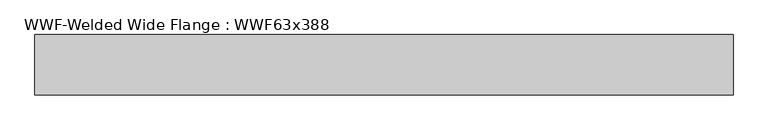
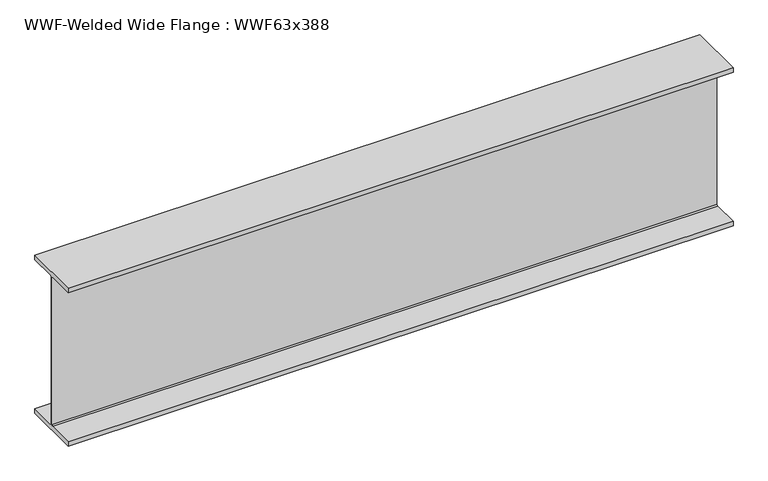
"""IFC4 building model written with IfcOpenShell, lengths in millimetres: beam geometry, WWF-Welded Wide Flange : WWF63x388."""

from ifc_helpers import new_model, si_unit, frame, origin, place, context, project, spatial, polyline, outline, extrude, source, transform, mapped, element, save


def wwf_welded_wide_flange_wwf63x388_8b4b7818(model_context):
    return source(origin(), model_context, "Body", "SweptSolid", [
        extrude(outline(polyline([(274.955, -755.015), (274.955, -799.973), (-274.955, -799.973), (-274.955, -755.015), (-19.05, -755.015), (-8.001, -743.966), (-8.001, 743.966), (-19.05, 755.015), (-274.955, 755.015), (-274.955, 799.973), (274.955, 799.973), (274.955, 755.015), (19.05, 755.015), (8.001, 743.966), (8.001, -743.966), (19.05, -755.015), (274.955, -755.015)])), frame((-3184.569859, 0.0, 0.0), z_axis=(1.0, 0.0, 0.0), x_axis=(0.0, 1.0, 0.0)), (0.0, 0.0, 1.0), 6369.1344444),
    ])


if __name__ == "__main__":
    model = new_model("IFC4")
    model_context = context("Model", 3, world=origin())
    ifc_project = project(units=[si_unit("LENGTHUNIT", "METRE", prefix="MILLI")], contexts=[model_context])
    site = spatial("IfcSite", under=ifc_project)
    building = spatial("IfcBuilding", under=site)
    placement = place(None, origin())
    wwf_welded_wide_flange_wwf63x388_shape = wwf_welded_wide_flange_wwf63x388_8b4b7818(model_context)
    element("IfcBeam", 1, ObjectType="WWF-Welded Wide Flange : WWF63x388", at=placement, inside=building, context=model_context, shape_type="MappedRepresentation", body=[
        mapped(wwf_welded_wide_flange_wwf63x388_shape, transform((0.0, 0.0, 0.0), x_axis=(1.0, 0.0, 0.0), y_axis=(0.0, 1.0, 0.0), z_axis=(0.0, 0.0, 1.0))),
    ])
    save(model, "model.ifc")

# Revit data of these elements
# Type "WWF-Welded Wide Flange : WWF63x388"
#   Assembly Code = "B10"
#   Nominal d = "12"
#   W = 388
#   Length [instance default] = 1524 mm
#   bf = 549.91 mm
#   d = 1599.946 mm
#   k = 19.05 mm
#   tf = 44.958 mm
#   tw = 16.002 mm
#   A = 0.0735482 m²
#   Structural Material [instance default] = Steel ASTM A572
# Element 1 (IfcBeam, "WWF-Welded Wide Flange : WWF63x388")
#   Structural Material = Metal - Steel 43-275
#   Materials on its faces: "Metal - Steel 43-275"
# Materials
#   "Steel ASTM A572": class "Metal", colour RGB 247 247 247, transparency 0, Description = "Structural steel, high strength low alloy, ASTM - A572 - 50", Cost = 0
#   "Metal - Steel 43-275": class "Metal", colour RGB 247 247 247, transparency 0, Cost = 0
